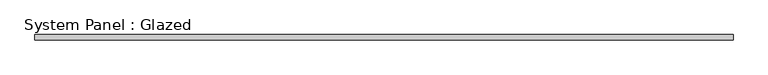
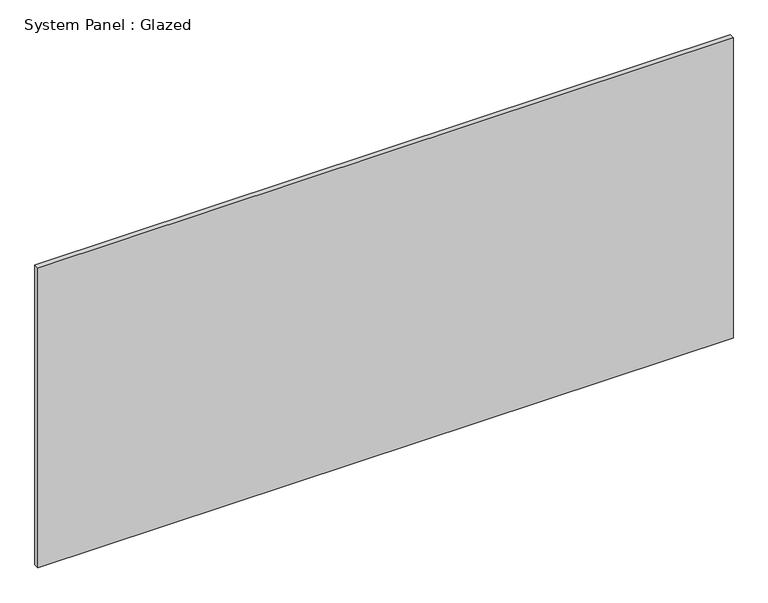
"""IFC4 building model written with IfcOpenShell, lengths in millimetres: plate geometry, System Panel : Glazed."""

from ifc_helpers import new_model, si_unit, origin, origin_with_axes, place, context, project, spatial, polyline, outline, extrude, source, transform, mapped, element, save


def system_panel_glazed_60e00337(model_context):
    return source(origin(), model_context, "Body", "SweptSolid", [
        extrude(outline(polyline([(1670.375, 24.5), (-1670.375, 24.5), (-1670.375, 49.5), (1670.375, 49.5), (1670.375, 24.5)])), origin_with_axes(), (0.0, 0.0, 1.0), 1526.020449),
    ])


if __name__ == "__main__":
    model = new_model("IFC4")
    model_context = context("Model", 3, world=origin())
    ifc_project = project(units=[si_unit("LENGTHUNIT", "METRE", prefix="MILLI")], contexts=[model_context])
    site = spatial("IfcSite", under=ifc_project)
    building = spatial("IfcBuilding", under=site)
    placement = place(None, origin())
    system_panel_glazed_shape = system_panel_glazed_60e00337(model_context)
    element("IfcPlate", 1, ObjectType="System Panel : Glazed", at=placement, inside=building, context=model_context, shape_type="MappedRepresentation", body=[
        mapped(system_panel_glazed_shape, transform((0.0, 0.0, 0.0), x_axis=(1.0, 0.0, 0.0), y_axis=(0.0, 1.0, 0.0), z_axis=(0.0, 0.0, 1.0))),
    ])
    save(model, "model.ifc")

# Revit data of these elements
# Type "System Panel : Glazed"
#   Keynote = "H11"
#   Construction Type Id = "GSP4R"
#   Analytic Construction = "1/8 in Pilkington single glazing"
#   Visual Light Transmittance = 0.9
#   Solar Heat Gain Coefficient = 0.86
#   Heat Transfer Coefficient (U) = 6.7069 W/(m²·K)
#   Define Thermal Properties by = 1
# Element 1 (IfcPlate, "System Panel : Glazed")
#   Materials on its faces: "Glass"
# Materials
#   "Glass": class "Glass", colour RGB 0 128 192, transparency 0.9, Description = "Soda Lime Glass", Cost = 0
